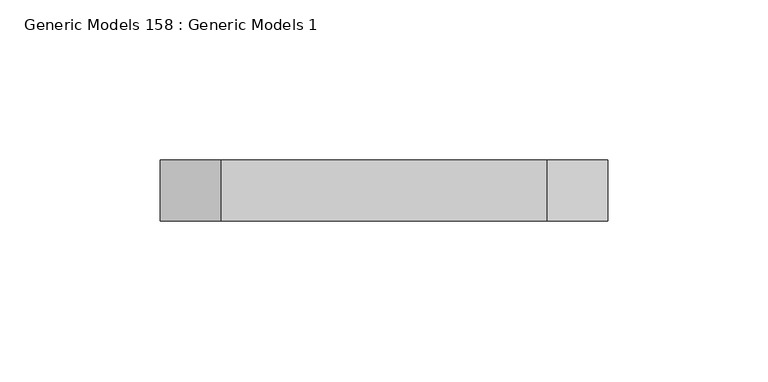
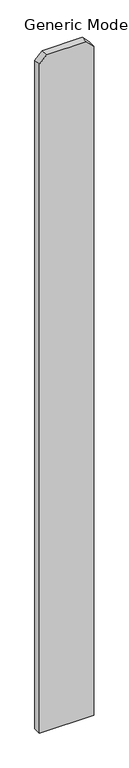
"""IFC4 building model written with IfcOpenShell, lengths in millimetres: proxy geometry, Generic Models 158 : Generic Models 1."""

import ifcopenshell
import ifcopenshell.guid

model = None  # the IFC model being written
_history = None  # IfcOwnerHistory: only IFC2X3 demands one
_inside = {}  # id of a spatial element -> (the spatial element, [elements in it])
_under = {}  # id of a project, library or spatial element -> (it, [spatial elements below it])
_declared = {}  # id of a project -> (the project, [libraries it declares])
_typed = {}  # id of a type object -> (the type object, [elements of that type])
_made_of = {}  # id of a material, layer set ... -> (it, [elements and type objects made of it])


def new_model(schema):
    """Start an empty IFC model of exactly this schema.

    Asked for "IFC4X3", IfcOpenShell would pick the latest addendum, in which some entities
    have other attributes; the version numbers below select the first issue.
    IFC2X3 requires an IfcOwnerHistory on every rooted entity: one is made here for all.
    """
    global model, _history
    if schema == "IFC4X3":
        model = ifcopenshell.file(schema_version=(4, 3, 0, 0))
    else:
        model = ifcopenshell.file(schema=schema)
    _inside.clear()
    _under.clear()
    _declared.clear()
    _typed.clear()
    _made_of.clear()
    _history = None
    if model.schema == "IFC2X3":
        org = make("IfcOrganization", Name="unknown")
        user = make(
            "IfcPersonAndOrganization",
            ThePerson=make("IfcPerson", FamilyName="unknown"),
            TheOrganization=org,
        )
        app = make(
            "IfcApplication",
            ApplicationDeveloper=org,
            Version="unknown",
            ApplicationFullName="unknown",
            ApplicationIdentifier="unknown",
        )
        _history = make(
            "IfcOwnerHistory",
            OwningUser=user,
            OwningApplication=app,
            ChangeAction="ADDED",
            CreationDate=0,
        )
    return model


def make(cls, **values):
    """One entity of the class cls with the attributes given. An attribute that is None is left unset."""
    return model.create_entity(
        cls, **{name: value for name, value in values.items() if value is not None}
    )


def rooted(cls, **values):
    """An entity with a GlobalId (a new one), such as an element, a storey or a relation."""
    return make(cls, GlobalId=ifcopenshell.guid.new(), OwnerHistory=_history, **values)


def si_unit(unit_type, name, prefix=None):
    """IfcSIUnit, for example si_unit("LENGTHUNIT", "METRE", prefix="MILLI")."""
    return make("IfcSIUnit", UnitType=unit_type, Prefix=prefix, Name=name)


def assignment(units):
    """IfcUnitAssignment: the units of a project."""
    return None if units is None else make("IfcUnitAssignment", Units=units)


def point(xyz):
    """IfcCartesianPoint."""
    return None if xyz is None else make("IfcCartesianPoint", Coordinates=xyz)


def direction(xyz):
    """IfcDirection."""
    return None if xyz is None else make("IfcDirection", DirectionRatios=xyz)


def frame(location, z_axis=None, x_axis=None):
    """IfcAxis2Placement3D, a coordinate frame: its origin and axes. An axis left out is left unset."""
    return make(
        "IfcAxis2Placement3D",
        Location=point(location),
        Axis=direction(z_axis),
        RefDirection=direction(x_axis),
    )


def origin():
    """The frame at (0, 0, 0) with its axes left unset."""
    return frame((0.0, 0.0, 0.0))


def place(relative_to, where):
    """IfcLocalPlacement: puts the frame where relative to a parent placement (None: the world)."""
    return make(
        "IfcLocalPlacement", PlacementRelTo=relative_to, RelativePlacement=where
    )


def context(
    kind, dimensions, precision=None, world=None, true_north=None, identifier=None
):
    """IfcGeometricRepresentationContext, for example the 3D "Model" context."""
    return make(
        "IfcGeometricRepresentationContext",
        ContextIdentifier=identifier,
        ContextType=kind,
        CoordinateSpaceDimension=dimensions,
        Precision=precision,
        WorldCoordinateSystem=world,
        TrueNorth=true_north,
    )


def project(units=None, contexts=None):
    """IfcProject with its units and contexts."""
    return rooted(
        "IfcProject",
        Name="project",
        RepresentationContexts=contexts,
        UnitsInContext=assignment(units),
    )


def spatial(cls, under=None, at=None, **own):
    """A site, building, storey or space (cls), placed at a placement, below another one or the project."""
    s = rooted(cls, ObjectPlacement=at, **own)
    if under is not None:
        _under.setdefault(under.id(), (under, []))[1].append(s)
    return s


def polyline(points):
    """IfcPolyline through the points."""
    return make("IfcPolyline", Points=[point(p) for p in points])


def outline(outer, holes=None, kind="AREA"):
    """IfcArbitraryClosedProfileDef: a profile drawn as a closed curve; with holes, ...WithVoids."""
    if holes is None:
        return make("IfcArbitraryClosedProfileDef", ProfileType=kind, OuterCurve=outer)
    return make(
        "IfcArbitraryProfileDefWithVoids",
        ProfileType=kind,
        OuterCurve=outer,
        InnerCurves=holes,
    )


def extrude(swept, where, along, depth):
    """IfcExtrudedAreaSolid: the profile swept, set in the frame where, extruded along a direction by depth."""
    return make(
        "IfcExtrudedAreaSolid",
        SweptArea=swept,
        Position=where,
        ExtrudedDirection=direction(along),
        Depth=depth,
    )


def shape(context_of_items, identifier, shape_type, items):
    """IfcShapeRepresentation: the items that make up one representation, for example the "Body"."""
    return make(
        "IfcShapeRepresentation",
        ContextOfItems=context_of_items,
        RepresentationIdentifier=identifier,
        RepresentationType=shape_type,
        Items=items,
    )


def source(mapping_origin, context_of_items, identifier, shape_type, items):
    """IfcRepresentationMap: a shape defined once, which mapped items show again and again."""
    return make(
        "IfcRepresentationMap",
        MappingOrigin=mapping_origin,
        MappedRepresentation=shape(context_of_items, identifier, shape_type, items),
    )


def transform(
    local_origin,
    x_axis=None,
    y_axis=None,
    z_axis=None,
    scale=None,
    scale2=None,
    scale3=None,
    uniform=True,
):
    """IfcCartesianTransformationOperator3D, or its non-uniform kind. x_axis, y_axis, z_axis: its Axis1, 2, 3."""
    if uniform:
        return make(
            "IfcCartesianTransformationOperator3D",
            Axis1=direction(x_axis),
            Axis2=direction(y_axis),
            LocalOrigin=point(local_origin),
            Scale=scale,
            Axis3=direction(z_axis),
        )
    return make(
        "IfcCartesianTransformationOperator3DnonUniform",
        Axis1=direction(x_axis),
        Axis2=direction(y_axis),
        LocalOrigin=point(local_origin),
        Scale=scale,
        Axis3=direction(z_axis),
        Scale2=scale2,
        Scale3=scale3,
    )


def mapped(mapping_source, mapping_target):
    """IfcMappedItem: shows the shape of a source again, moved by a transform."""
    return make(
        "IfcMappedItem", MappingSource=mapping_source, MappingTarget=mapping_target
    )


def made_of(thing, what):
    """Note that an element or type object is made of a material, layer set ...; save() writes the relation."""
    if what is not None:
        _made_of.setdefault(what.id(), (what, []))[1].append(thing)
    return thing


def element(
    cls,
    number,
    at=None,
    inside=None,
    cuts=None,
    type_object=None,
    material=None,
    context=None,
    identifier="Body",
    shape_type=None,
    held_by="IfcProductDefinitionShape",
    body=None,
    shapes=None,
    **own,
):
    """One element of the class cls, such as IfcWall. Its Tag is "e" and its number.

    at: its placement. inside: the storey or other place that contains it. cuts: it is an
    opening in that element (IfcRelVoidsElement). A single representation is given by context,
    identifier, shape_type and body (its items); several are given by shapes. held_by: the class
    of the entity that holds the representations. save() writes the other relations.
    """
    e = rooted(cls, Tag="e%d" % number, ObjectPlacement=at, **own)
    if body is not None:
        shapes = [shape(context, identifier, shape_type, body)]
    if shapes is not None:
        e.Representation = make(held_by, Representations=shapes)
    if inside is not None:
        _inside.setdefault(inside.id(), (inside, []))[1].append(e)
    if cuts is not None:
        rooted(
            "IfcRelVoidsElement", RelatingBuildingElement=cuts, RelatedOpeningElement=e
        )
    if type_object is not None:
        _typed.setdefault(type_object.id(), (type_object, []))[1].append(e)
    return made_of(e, material)


def aggregate(whole, parts):
    """IfcRelAggregates: a whole, such as a stair, and the parts it consists of."""
    return rooted("IfcRelAggregates", RelatingObject=whole, RelatedObjects=parts)


def save(model, path):
    """Write the relations noted so far, then the file.

    IfcRelAggregates (storeys below a building ...), IfcRelContainedInSpatialStructure (elements
    in a storey), IfcRelDefinesByType, IfcRelAssociatesMaterial and IfcRelDeclares: one each for
    every whole, place, type object, material and project.
    """
    for whole, parts in _under.values():
        aggregate(whole, parts)
    for where, things in _inside.values():
        rooted(
            "IfcRelContainedInSpatialStructure",
            RelatedElements=things,
            RelatingStructure=where,
        )
    for kind, things in _typed.values():
        rooted("IfcRelDefinesByType", RelatedObjects=things, RelatingType=kind)
    for what, things in _made_of.values():
        rooted("IfcRelAssociatesMaterial", RelatedObjects=things, RelatingMaterial=what)
    for by, libraries in _declared.values():
        rooted("IfcRelDeclares", RelatingContext=by, RelatedDefinitions=libraries)
    model.write(path)


def generic_models_158_generic_models_1_4ff7d1c7(model_context):
    return source(origin(), model_context, "Body", "SweptSolid", [
        extrude(outline(polyline([(76.2, 54075.0125), (1885.95, 54075.0125), (1905.0, 54055.9625), (1905.0, 53954.3625), (1885.95, 53935.3125), (76.2, 53935.3125), (76.2, 54075.0125)])), frame((0.0, 547.6875, 0.0), z_axis=(0.0, 1.0, 0.0), x_axis=(0.0, 0.0, 1.0)), (0.0, 0.0, 1.0), 19.05),
    ])


if __name__ == "__main__":
    model = new_model("IFC4")
    model_context = context("Model", 3, world=origin())
    ifc_project = project(units=[si_unit("LENGTHUNIT", "METRE", prefix="MILLI")], contexts=[model_context])
    site = spatial("IfcSite", under=ifc_project)
    building = spatial("IfcBuilding", under=site)
    placement = place(None, origin())
    generic_models_158_generic_models_1_shape = generic_models_158_generic_models_1_4ff7d1c7(model_context)
    element("IfcBuildingElementProxy", 1, Name="Generic Models 158 : Generic Models 1", ObjectType="Generic Models 158 : Generic Models 1", at=placement, inside=building, context=model_context, shape_type="MappedRepresentation", body=[
        mapped(generic_models_158_generic_models_1_shape, transform((0.0, 0.0, 0.0), x_axis=(1.0, 0.0, 0.0), y_axis=(0.0, 1.0, 0.0), z_axis=(0.0, 0.0, 1.0))),
    ])
    save(model, "model.ifc")

# Revit data of these elements
# Element 1 (IfcBuildingElementProxy, "Generic Models 158 : Generic Models 1")
#   Materials on its faces: "VERTICAL 1X6 CEDAR PLANKS W/ CLEAR WOOD SEALER"
# Materials
#   "VERTICAL 1X6 CEDAR PLANKS W/ CLEAR WOOD SEALER": class "Wood", colour RGB 234 198 147, transparency 0, Description = "Pinus Echinata", Cost = 0
